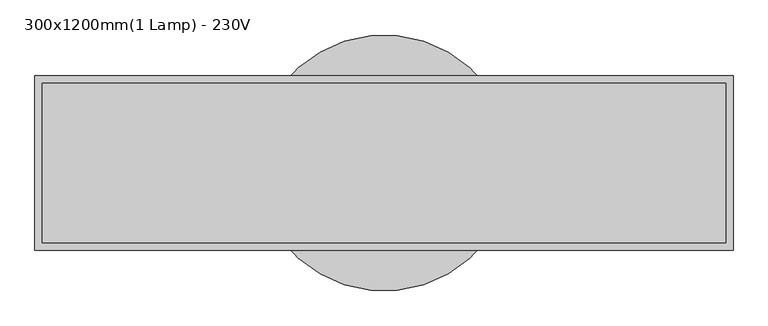
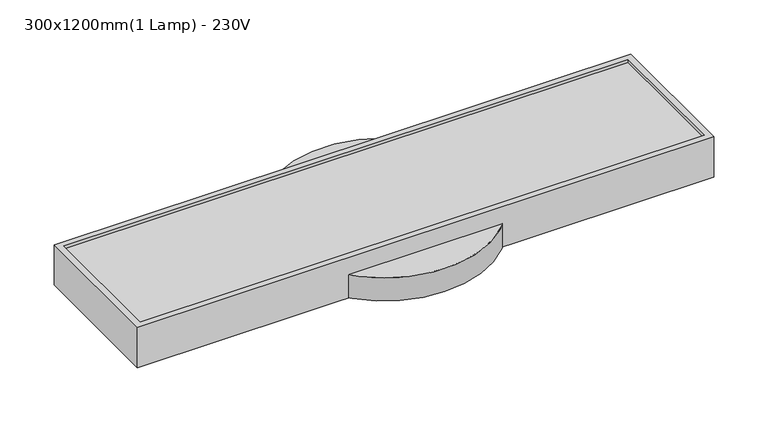
"""IFC4 building model written with IfcOpenShell, lengths in millimetres: light fixture geometry, Ceiling Light - Linear Box emergency light 300x1200mm 1Lamp 230 v : 300x1200mm(1 Lamp) - 230V."""

import ifcopenshell
import ifcopenshell.guid

model = None  # the IFC model being written
_history = None  # IfcOwnerHistory: only IFC2X3 demands one
_inside = {}  # id of a spatial element -> (the spatial element, [elements in it])
_under = {}  # id of a project, library or spatial element -> (it, [spatial elements below it])
_declared = {}  # id of a project -> (the project, [libraries it declares])
_typed = {}  # id of a type object -> (the type object, [elements of that type])
_made_of = {}  # id of a material, layer set ... -> (it, [elements and type objects made of it])


def new_model(schema):
    """Start an empty IFC model of exactly this schema.

    Asked for "IFC4X3", IfcOpenShell would pick the latest addendum, in which some entities
    have other attributes; the version numbers below select the first issue.
    IFC2X3 requires an IfcOwnerHistory on every rooted entity: one is made here for all.
    """
    global model, _history
    if schema == "IFC4X3":
        model = ifcopenshell.file(schema_version=(4, 3, 0, 0))
    else:
        model = ifcopenshell.file(schema=schema)
    _inside.clear()
    _under.clear()
    _declared.clear()
    _typed.clear()
    _made_of.clear()
    _history = None
    if model.schema == "IFC2X3":
        org = make("IfcOrganization", Name="unknown")
        user = make(
            "IfcPersonAndOrganization",
            ThePerson=make("IfcPerson", FamilyName="unknown"),
            TheOrganization=org,
        )
        app = make(
            "IfcApplication",
            ApplicationDeveloper=org,
            Version="unknown",
            ApplicationFullName="unknown",
            ApplicationIdentifier="unknown",
        )
        _history = make(
            "IfcOwnerHistory",
            OwningUser=user,
            OwningApplication=app,
            ChangeAction="ADDED",
            CreationDate=0,
        )
    return model


def make(cls, **values):
    """One entity of the class cls with the attributes given. An attribute that is None is left unset."""
    return model.create_entity(
        cls, **{name: value for name, value in values.items() if value is not None}
    )


def rooted(cls, **values):
    """An entity with a GlobalId (a new one), such as an element, a storey or a relation."""
    return make(cls, GlobalId=ifcopenshell.guid.new(), OwnerHistory=_history, **values)


def si_unit(unit_type, name, prefix=None):
    """IfcSIUnit, for example si_unit("LENGTHUNIT", "METRE", prefix="MILLI")."""
    return make("IfcSIUnit", UnitType=unit_type, Prefix=prefix, Name=name)


def assignment(units):
    """IfcUnitAssignment: the units of a project."""
    return None if units is None else make("IfcUnitAssignment", Units=units)


def point(xyz):
    """IfcCartesianPoint."""
    return None if xyz is None else make("IfcCartesianPoint", Coordinates=xyz)


def direction(xyz):
    """IfcDirection."""
    return None if xyz is None else make("IfcDirection", DirectionRatios=xyz)


def frame(location, z_axis=None, x_axis=None):
    """IfcAxis2Placement3D, a coordinate frame: its origin and axes. An axis left out is left unset."""
    return make(
        "IfcAxis2Placement3D",
        Location=point(location),
        Axis=direction(z_axis),
        RefDirection=direction(x_axis),
    )


def frame_2d(location, x_axis=None):
    """IfcAxis2Placement2D, a coordinate frame in the plane: its origin and x axis."""
    return make(
        "IfcAxis2Placement2D", Location=point(location), RefDirection=direction(x_axis)
    )


def origin():
    """The frame at (0, 0, 0) with its axes left unset."""
    return frame((0.0, 0.0, 0.0))


def origin_with_axes():
    """The frame at (0, 0, 0) with the z axis (0, 0, 1) and the x axis (1, 0, 0) written out."""
    return frame((0.0, 0.0, 0.0), z_axis=(0.0, 0.0, 1.0), x_axis=(1.0, 0.0, 0.0))


def place(relative_to, where):
    """IfcLocalPlacement: puts the frame where relative to a parent placement (None: the world)."""
    return make(
        "IfcLocalPlacement", PlacementRelTo=relative_to, RelativePlacement=where
    )


def context(
    kind, dimensions, precision=None, world=None, true_north=None, identifier=None
):
    """IfcGeometricRepresentationContext, for example the 3D "Model" context."""
    return make(
        "IfcGeometricRepresentationContext",
        ContextIdentifier=identifier,
        ContextType=kind,
        CoordinateSpaceDimension=dimensions,
        Precision=precision,
        WorldCoordinateSystem=world,
        TrueNorth=true_north,
    )


def project(units=None, contexts=None):
    """IfcProject with its units and contexts."""
    return rooted(
        "IfcProject",
        Name="project",
        RepresentationContexts=contexts,
        UnitsInContext=assignment(units),
    )


def spatial(cls, under=None, at=None, **own):
    """A site, building, storey or space (cls), placed at a placement, below another one or the project."""
    s = rooted(cls, ObjectPlacement=at, **own)
    if under is not None:
        _under.setdefault(under.id(), (under, []))[1].append(s)
    return s


def polyline(points):
    """IfcPolyline through the points."""
    return make("IfcPolyline", Points=[point(p) for p in points])


def circle_curve(where, radius):
    """IfcCircle in the frame where."""
    return make("IfcCircle", Position=where, Radius=radius)


def trimmed(basis, trim1, trim2, sense, master):
    """IfcTrimmedCurve: the piece of a basis curve between two trims."""
    return make(
        "IfcTrimmedCurve",
        BasisCurve=basis,
        Trim1=trim1,
        Trim2=trim2,
        SenseAgreement=sense,
        MasterRepresentation=master,
    )


def segment(curve, same_sense, transition):
    """IfcCompositeCurveSegment."""
    return make(
        "IfcCompositeCurveSegment",
        Transition=transition,
        SameSense=same_sense,
        ParentCurve=curve,
    )


def composite_curve(segments, self_intersect=None):
    """IfcCompositeCurve: segments joined end to end."""
    return make("IfcCompositeCurve", Segments=segments, SelfIntersect=self_intersect)


def outline(outer, holes=None, kind="AREA"):
    """IfcArbitraryClosedProfileDef: a profile drawn as a closed curve; with holes, ...WithVoids."""
    if holes is None:
        return make("IfcArbitraryClosedProfileDef", ProfileType=kind, OuterCurve=outer)
    return make(
        "IfcArbitraryProfileDefWithVoids",
        ProfileType=kind,
        OuterCurve=outer,
        InnerCurves=holes,
    )


def extrude(swept, where, along, depth):
    """IfcExtrudedAreaSolid: the profile swept, set in the frame where, extruded along a direction by depth."""
    return make(
        "IfcExtrudedAreaSolid",
        SweptArea=swept,
        Position=where,
        ExtrudedDirection=direction(along),
        Depth=depth,
    )


def shape(context_of_items, identifier, shape_type, items):
    """IfcShapeRepresentation: the items that make up one representation, for example the "Body"."""
    return make(
        "IfcShapeRepresentation",
        ContextOfItems=context_of_items,
        RepresentationIdentifier=identifier,
        RepresentationType=shape_type,
        Items=items,
    )


def source(mapping_origin, context_of_items, identifier, shape_type, items):
    """IfcRepresentationMap: a shape defined once, which mapped items show again and again."""
    return make(
        "IfcRepresentationMap",
        MappingOrigin=mapping_origin,
        MappedRepresentation=shape(context_of_items, identifier, shape_type, items),
    )


def transform(
    local_origin,
    x_axis=None,
    y_axis=None,
    z_axis=None,
    scale=None,
    scale2=None,
    scale3=None,
    uniform=True,
):
    """IfcCartesianTransformationOperator3D, or its non-uniform kind. x_axis, y_axis, z_axis: its Axis1, 2, 3."""
    if uniform:
        return make(
            "IfcCartesianTransformationOperator3D",
            Axis1=direction(x_axis),
            Axis2=direction(y_axis),
            LocalOrigin=point(local_origin),
            Scale=scale,
            Axis3=direction(z_axis),
        )
    return make(
        "IfcCartesianTransformationOperator3DnonUniform",
        Axis1=direction(x_axis),
        Axis2=direction(y_axis),
        LocalOrigin=point(local_origin),
        Scale=scale,
        Axis3=direction(z_axis),
        Scale2=scale2,
        Scale3=scale3,
    )


def mapped(mapping_source, mapping_target):
    """IfcMappedItem: shows the shape of a source again, moved by a transform."""
    return make(
        "IfcMappedItem", MappingSource=mapping_source, MappingTarget=mapping_target
    )


def made_of(thing, what):
    """Note that an element or type object is made of a material, layer set ...; save() writes the relation."""
    if what is not None:
        _made_of.setdefault(what.id(), (what, []))[1].append(thing)
    return thing


def element(
    cls,
    number,
    at=None,
    inside=None,
    cuts=None,
    type_object=None,
    material=None,
    context=None,
    identifier="Body",
    shape_type=None,
    held_by="IfcProductDefinitionShape",
    body=None,
    shapes=None,
    **own,
):
    """One element of the class cls, such as IfcWall. Its Tag is "e" and its number.

    at: its placement. inside: the storey or other place that contains it. cuts: it is an
    opening in that element (IfcRelVoidsElement). A single representation is given by context,
    identifier, shape_type and body (its items); several are given by shapes. held_by: the class
    of the entity that holds the representations. save() writes the other relations.
    """
    e = rooted(cls, Tag="e%d" % number, ObjectPlacement=at, **own)
    if body is not None:
        shapes = [shape(context, identifier, shape_type, body)]
    if shapes is not None:
        e.Representation = make(held_by, Representations=shapes)
    if inside is not None:
        _inside.setdefault(inside.id(), (inside, []))[1].append(e)
    if cuts is not None:
        rooted(
            "IfcRelVoidsElement", RelatingBuildingElement=cuts, RelatedOpeningElement=e
        )
    if type_object is not None:
        _typed.setdefault(type_object.id(), (type_object, []))[1].append(e)
    return made_of(e, material)


def aggregate(whole, parts):
    """IfcRelAggregates: a whole, such as a stair, and the parts it consists of."""
    return rooted("IfcRelAggregates", RelatingObject=whole, RelatedObjects=parts)


def save(model, path):
    """Write the relations noted so far, then the file.

    IfcRelAggregates (storeys below a building ...), IfcRelContainedInSpatialStructure (elements
    in a storey), IfcRelDefinesByType, IfcRelAssociatesMaterial and IfcRelDeclares: one each for
    every whole, place, type object, material and project.
    """
    for whole, parts in _under.values():
        aggregate(whole, parts)
    for where, things in _inside.values():
        rooted(
            "IfcRelContainedInSpatialStructure",
            RelatedElements=things,
            RelatingStructure=where,
        )
    for kind, things in _typed.values():
        rooted("IfcRelDefinesByType", RelatedObjects=things, RelatingType=kind)
    for what, things in _made_of.values():
        rooted("IfcRelAssociatesMaterial", RelatedObjects=things, RelatingMaterial=what)
    for by, libraries in _declared.values():
        rooted("IfcRelDeclares", RelatingContext=by, RelatedDefinitions=libraries)
    model.write(path)


def light_fixture_300x1200mm_1_lamp_230v_5a723bfd(model_context):
    return source(origin(), model_context, "Body", "SweptSolid", [
        extrude(outline(composite_curve([segment(trimmed(circle_curve(frame_2d((0.0, -150.0)), 220.0), [point((-220.0, -150.0))], [point((220.0, -150.0))], False, "CARTESIAN"), True, "CONTINUOUS"), segment(trimmed(circle_curve(frame_2d((0.0, -150.0)), 220.0), [point((220.0, -150.0))], [point((-220.0, -150.0))], False, "CARTESIAN"), True, "CONTINUOUS")], self_intersect=False)), origin_with_axes(), (0.0, 0.0, 1.0), 50.8),
        extrude(outline(polyline([(587.3, -12.7), (587.3, -287.3), (-587.3, -287.3), (-587.3, -12.7), (587.3, -12.7)])), frame((0.0, 0.0, 76.2), z_axis=(0.0, 0.0, 1.0), x_axis=(1.0, 0.0, 0.0)), (0.0, 0.0, 1.0), 6.35),
        extrude(outline(polyline([(600.0, 0.0), (600.0, -300.0), (-600.0, -300.0), (-600.0, 0.0), (600.0, 0.0)]), holes=[polyline([(587.3, -12.7), (-587.3, -12.7), (-587.3, -287.3), (587.3, -287.3), (587.3, -12.7)])]), origin_with_axes(), (0.0, 0.0, 1.0), 88.9),
    ])


if __name__ == "__main__":
    model = new_model("IFC4")
    model_context = context("Model", 3, world=origin())
    ifc_project = project(units=[si_unit("LENGTHUNIT", "METRE", prefix="MILLI")], contexts=[model_context])
    site = spatial("IfcSite", under=ifc_project)
    building = spatial("IfcBuilding", under=site)
    placement = place(None, origin())
    light_fixture_300x1200mm_1_lamp_230v_shape = light_fixture_300x1200mm_1_lamp_230v_5a723bfd(model_context)
    element("IfcLightFixture", 1, ObjectType="Ceiling Light - Linear Box emergency light 300x1200mm 1Lamp 230 v : 300x1200mm(1 Lamp) - 230V", at=placement, inside=building, context=model_context, shape_type="MappedRepresentation", body=[
        mapped(light_fixture_300x1200mm_1_lamp_230v_shape, transform((0.0, 0.0, 0.0), x_axis=(1.0, 0.0, 0.0), y_axis=(0.0, 1.0, 0.0), z_axis=(0.0, 0.0, 1.0))),
    ])
    save(model, "model.ifc")

# Revit data of these elements
# Type "Ceiling Light - Linear Box emergency light 300x1200mm 1Lamp 230 v : 300x1200mm(1 Lamp) - 230V"
#   Type Mark = "Ceiling Light - Linear Box emergency light 300x1200mm 1Lamp 230 v"
#   Classification.OmniClass.21.Number = "21-04 50 40 50"
#   Classification.OmniClass.21.Description = "Lighting Fixtures"
#   Classification.UniFormat.II.Description = "Lighting Fixtures"
#   Classification.OmniClass.23.Number = "23-35 47 13"
#   Classification.OmniClass.23.Description = "Emergency Lighting"
#   Classification.UniFormat.II.Number = "D5040.50"
#   COBie.Type.CreatedBy = "info@mma.ie"
#   COBie.Type.CreatedOn = "2017-07-25T10:15:16"
#   COBie.Type.Name = "Ceiling Light - Linear Box emergency light 300x1200mm 1Lamp 230 v"
#   COBie.Type.Category = "23-35 47 13 : Emergency Lighting"
#   COBie.Type.Description = "Ceiling Light - Linear Box emergency light 300x1200mm 1Lamp 230 v_300x1200mm(1 Lamp) - 230V"
#   COBie.Type.AssetType = "Fixed"
#   COBie.Type.Manufacturer = ""
#   COBie.Type.ModelNumber = ""
#   Photometric Web File = "1x41T12.ies"
#   Lamp = "T-12"
#   Keynote = "26 52 00.A"
#   Assembly Code = "D5020210"
#   COBie.Type.ReplacementCost = 0
#   Width 1 = 150 mm
#   Wattage = 40 W
#   built-in parameter 1150110 = 1 (stored number, unit not read)
#   built-in parameter 1114217 = 0.88 (stored number, unit not read)
#   built-in parameter 1150109 = 1 (stored number, unit not read)
#   built-in parameter 1150113 = 1 (stored number, unit not read)
#   Tilt Angle = -90.00°
#   Lumens = 3150 lm
#   built-in parameter 1150115 = 1 (stored number, unit not read)
#   built-in parameter 1150105 = 250.669 (stored number, unit not read)
#   Length1 = 600 mm
#   built-in parameter 1150112 = 1 (stored number, unit not read)
#   built-in parameter 1150114 = 1 (stored number, unit not read)
#   built-in parameter 1150107 = 4230 (stored number, unit not read)
#   built-in parameter 1150106 = 2.50669 (stored number, unit not read)
#   Emit from Rectangle Width = 274 mm
#   Emit from Rectangle Length = 1174 mm
#   built-in parameter 1150104 = 7.31611 (stored number, unit not read)
#   Default Elevation = 1200 mm
#   C.L.E - Width = 300 mm
#   C.L.E - Length = 1200 mm
#   C.L.E - Depth = 88.9 mm
#   Box Width = 300 mm
#   Box Length = 1200 mm
#   Ballast Voltage = 230 V
#   built-in parameter 1114218 = 0.88 (stored number, unit not read)
#   built-in parameter 1150133 = 10 (stored number, unit not read)
#   Apparent Load = 40 VA
#   COBie.Type = yes
#   built-in parameter 1150134 = 8
#   built-in parameter 1150137 = 1
#   Color Filter = 16777215
#   built-in parameter 1140040 [instance default] = 1
#   Ballast Number of Poles = 1
#   black = Phase - Demo
#   Load Classification = Lighting - Dwelling Unit
#   Light Box Material = Metal - Paint Finish - Ivory, Glossy
#   Diffuser Material = Glass - White, High Luminance
#   Emit Shape Visible in Rendering = no
#   Dimming Lamp Color Temperature Shift = (empty or 0)
# Element 1 (IfcLightFixture, "Ceiling Light - Linear Box emergency light 300x1200mm 1Lamp 230 v : 300x1200mm(1 Lamp) - 230V")
#   Materials on its faces: "Phase - Demo", "Glass - White, High Luminance"
# Materials
#   "Phase - Demo": class "System", colour RGB 255 0 0, transparency 0.4
#   "Metal - Paint Finish - Ivory, Glossy": class "Paint", colour RGB 247 247 239, transparency 0, Comments = "Rendering appearance not upgraded "
#   "Glass - White, High Luminance": class "Glass", colour RGB 249 250 249, transparency 0.8
